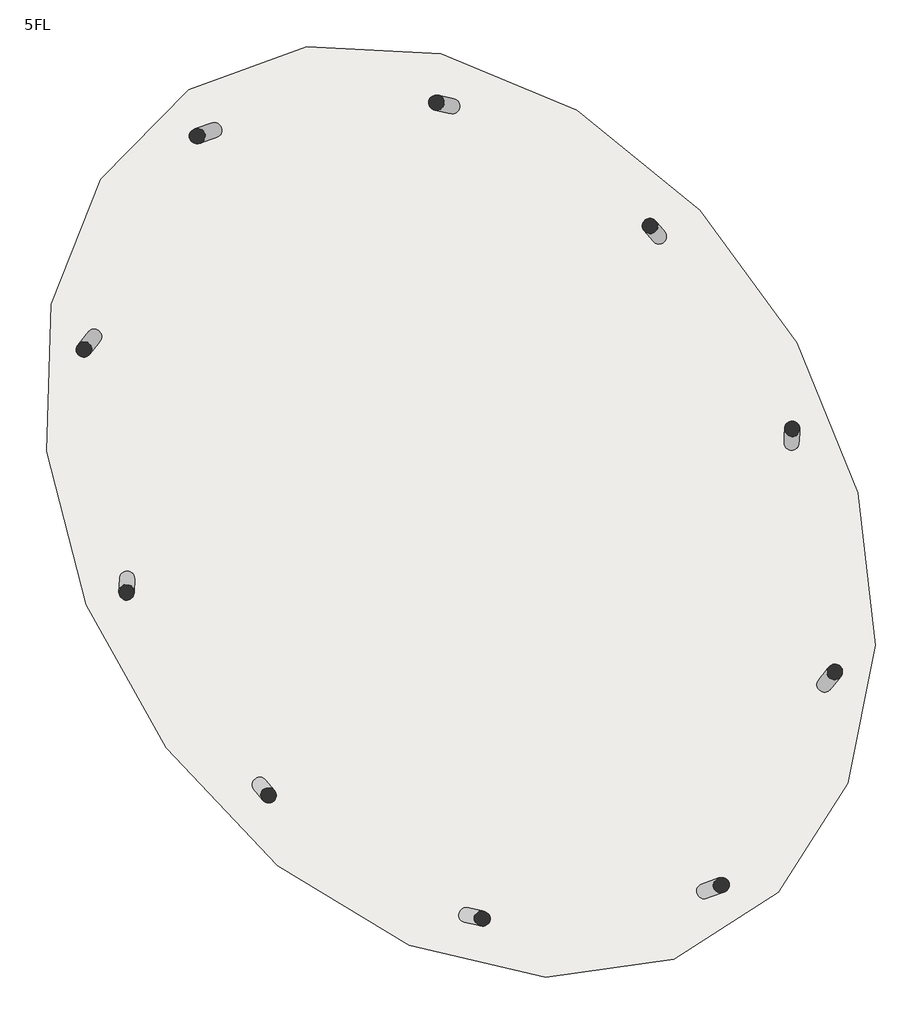
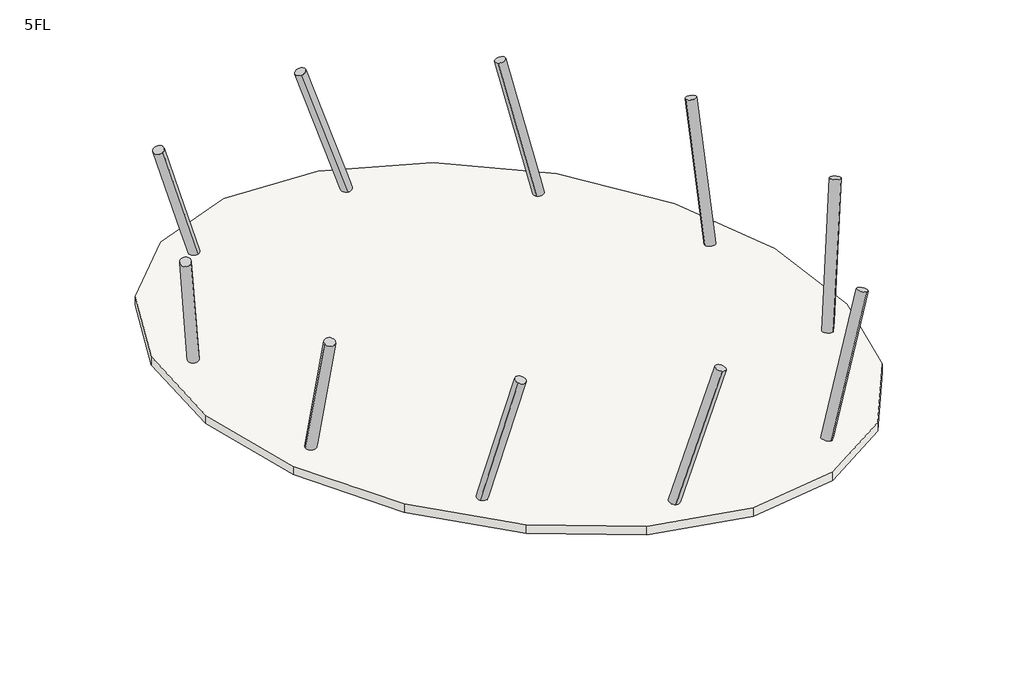
# One storey: 10 columns, 1 slab.
"""IFC4 building model written with IfcOpenShell, lengths in millimetres."""

from ifc_helpers import new_model, si_unit, point, frame, frame_2d, origin, place, context, project, spatial, polyline, circle_curve, trimmed, segment, composite_curve, outline, extrude, element, save

model = new_model("IFC4")

# Units and contexts
model_context = context("Model", 3, world=origin())
ifc_project = project(units=[si_unit("LENGTHUNIT", "METRE", prefix="MILLI")], contexts=[model_context])

# Site, building, storey
site = spatial("IfcSite", under=ifc_project)
building = spatial("IfcBuilding", under=site)
storey = spatial("IfcBuildingStorey", under=building, Name="5FL", Elevation=18000.0)

# Columns
placement = place(None, origin())
element("IfcColumn", 1, ObjectType="コンクリート-円形-柱 : 750", at=placement, inside=storey, context=model_context, shape_type="SweptSolid", body=[
    extrude(outline(composite_curve([segment(trimmed(circle_curve(frame_2d((0.0, -175.0000001)), 175.0), [point((0.0, -350.0000001))], [point((0.0, 0.0))], False, "CARTESIAN"), True, "CONTINUOUS"), segment(trimmed(circle_curve(frame_2d((0.0, -175.0000001)), 175.0), [point((0.0, 0.0))], [point((0.0, -350.0000001))], False, "CARTESIAN"), True, "CONTINUOUS")], self_intersect=False)), frame((-5595.8820356, 8632.5549364, 18000.0), z_axis=(-0.3160724442393226, -0.11108929791393882, 0.9422087761645868), x_axis=(-0.8889040361904681, -0.31242117778067396, -0.3350263006368777)), (0.0, 0.0, 1.0), 4776.0115527),
])
element("IfcColumn", 2, ObjectType="コンクリート-円形-柱 : 750", at=placement, inside=storey, context=model_context, shape_type="SweptSolid", body=[
    extrude(outline(composite_curve([segment(trimmed(circle_curve(frame_2d((0.0, -175.0)), 175.0), [point((0.0, -350.0))], [point((0.0, 0.0))], False, "CARTESIAN"), True, "CONTINUOUS"), segment(trimmed(circle_curve(frame_2d((0.0, -175.0)), 175.0), [point((0.0, 0.0))], [point((0.0, -350.0))], False, "CARTESIAN"), True, "CONTINUOUS")], self_intersect=False)), frame((-8300.1966174, 3915.2551119, 18000.0), z_axis=(-0.19134437507856675, -0.23607455338716757, 0.952709890453984), x_axis=(-0.5998910059272748, -0.7401262840734711, -0.3038813331403524)), (0.0, 0.0, 1.0), 4723.3686194),
])
element("IfcColumn", 3, ObjectType="コンクリート-円形-柱 : 750", at=placement, inside=storey, context=model_context, shape_type="SweptSolid", body=[
    extrude(outline(composite_curve([segment(trimmed(circle_curve(frame_2d((0.0, -174.9999999)), 175.0), [point((1e-07, -350.0))], [point((0.0, 0.0))], False, "CARTESIAN"), True, "CONTINUOUS"), segment(trimmed(circle_curve(frame_2d((0.0, -174.9999999)), 175.0), [point((0.0, 0.0))], [point((1e-07, -350.0))], False, "CARTESIAN"), True, "CONTINUOUS")], self_intersect=False)), frame((-7503.5385113, -1574.7884735, 18000.0), z_axis=(-0.010174401539469679, -0.2585133773793969, 0.9659540958395545), x_axis=(-0.037987983353784824, -0.9652068319225283, -0.25871351864714925)), (0.0, 0.0, 1.0), 4658.6064694),
])
element("IfcColumn", 4, ObjectType="コンクリート-円形-柱 : 750", at=placement, inside=storey, context=model_context, shape_type="SweptSolid", body=[
    extrude(outline(composite_curve([segment(trimmed(circle_curve(frame_2d((1e-07, -175.0)), 175.0), [point((0.0, -350.0))], [point((0.0, 0.0))], False, "CARTESIAN"), True, "CONTINUOUS"), segment(trimmed(circle_curve(frame_2d((1e-07, -175.0)), 175.0), [point((0.0, 0.0))], [point((0.0, -350.0))], False, "CARTESIAN"), True, "CONTINUOUS")], self_intersect=False)), frame((-4481.951061, -6220.6214896, 18000.0), z_axis=(0.16585051662713518, -0.19741327886939466, 0.9661892172139714), x_axis=(0.6214965858800432, -0.7397726658913514, -0.25783404844871255)), (0.0, 0.0, 1.0), 4657.4727984),
])
element("IfcColumn", 5, ObjectType="コンクリート-円形-柱 : 750", at=placement, inside=storey, context=model_context, shape_type="SweptSolid", body=[
    extrude(outline(composite_curve([segment(trimmed(circle_curve(frame_2d((-1e-07, -174.9999999)), 175.0), [point((0.0, -349.9999999))], [point((0.0, 0.0))], False, "CARTESIAN"), True, "CONTINUOUS"), segment(trimmed(circle_curve(frame_2d((-1e-07, -174.9999999)), 175.0), [point((0.0, 0.0))], [point((0.0, -349.9999999))], False, "CARTESIAN"), True, "CONTINUOUS")], self_intersect=False)), frame((195.5067974, -9175.2712794, 18000.0), z_axis=(0.2953258471996599, -0.06630137645773637, 0.9530932648254382), x_axis=(0.9299460730744334, -0.20877517244407529, -0.302676772389933)), (0.0, 0.0, 1.0), 4721.4686802),
])
element("IfcColumn", 6, ObjectType="コンクリート-円形-柱 : 750", at=placement, inside=storey, context=model_context, shape_type="SweptSolid", body=[
    extrude(outline(composite_curve([segment(trimmed(circle_curve(frame_2d((0.0, -175.0000001)), 175.0), [point((0.0, -350.0))], [point((0.0, 0.0))], False, "CARTESIAN"), True, "CONTINUOUS"), segment(trimmed(circle_curve(frame_2d((0.0, -175.0000001)), 175.0), [point((0.0, 0.0))], [point((0.0, -350.0))], False, "CARTESIAN"), True, "CONTINUOUS")], self_intersect=False)), frame((5595.8820724, -8632.5549329, 18000.0), z_axis=(0.3160724441365904, 0.11108929887426984, 0.9422087760858234), x_axis=(0.888904035239524, 0.3124211802487731, -0.3350263008583877)), (0.0, 0.0, 1.0), 4776.0115527),
])
element("IfcColumn", 7, ObjectType="コンクリート-円形-柱 : 750", at=placement, inside=storey, context=model_context, shape_type="SweptSolid", body=[
    extrude(outline(composite_curve([segment(trimmed(circle_curve(frame_2d((0.0, -175.0)), 175.0), [point((0.0, -350.0))], [point((0.0, 0.0))], False, "CARTESIAN"), True, "CONTINUOUS"), segment(trimmed(circle_curve(frame_2d((0.0, -175.0)), 175.0), [point((0.0, 0.0))], [point((0.0, -350.0))], False, "CARTESIAN"), True, "CONTINUOUS")], self_intersect=False)), frame((8300.1966113, -3915.2550865, 18000.0), z_axis=(0.19134437572990706, 0.23607455280450085, 0.9527098904675481), x_axis=(0.5998910080618053, 0.7401262823608402, -0.3038813330978276)), (0.0, 0.0, 1.0), 4723.3686194),
])
element("IfcColumn", 8, ObjectType="コンクリート-円形-柱 : 750", at=placement, inside=storey, context=model_context, shape_type="SweptSolid", body=[
    extrude(outline(composite_curve([segment(trimmed(circle_curve(frame_2d((0.0, -175.0)), 175.0), [point((0.0, -350.0000001))], [point((0.0, 0.0))], False, "CARTESIAN"), True, "CONTINUOUS"), segment(trimmed(circle_curve(frame_2d((0.0, -175.0)), 175.0), [point((0.0, 0.0))], [point((0.0, -350.0000001))], False, "CARTESIAN"), True, "CONTINUOUS")], self_intersect=False)), frame((7503.5384883, 1574.7884899, 18000.0), z_axis=(0.01017440149479294, 0.2585133764783915, 0.9659540960811566), x_axis=(0.03798798332893155, 0.9652068321652956, -0.25871351774508383)), (0.0, 0.0, 1.0), 4658.6064694),
])
element("IfcColumn", 9, ObjectType="コンクリート-円形-柱 : 750", at=placement, inside=storey, context=model_context, shape_type="SweptSolid", body=[
    extrude(outline(composite_curve([segment(trimmed(circle_curve(frame_2d((0.0, -175.0)), 175.0), [point((0.0, -350.0000001))], [point((0.0, 0.0))], False, "CARTESIAN"), True, "CONTINUOUS"), segment(trimmed(circle_curve(frame_2d((0.0, -175.0)), 175.0), [point((0.0, 0.0))], [point((0.0, -350.0000001))], False, "CARTESIAN"), True, "CONTINUOUS")], self_intersect=False)), frame((4481.95109, 6220.6214639, 18000.0), z_axis=(-0.16585051382729254, 0.19741327854709606, 0.9661892177604291), x_axis=(-0.6214965806756345, 0.7397726709773783, -0.2578340464009559)), (0.0, 0.0, 1.0), 4657.4727984),
])
element("IfcColumn", 10, ObjectType="コンクリート-円形-柱 : 750", at=placement, inside=storey, context=model_context, shape_type="SweptSolid", body=[
    extrude(outline(composite_curve([segment(trimmed(circle_curve(frame_2d((1e-07, -175.0)), 175.0), [point((0.0, -350.0))], [point((0.0, 0.0))], False, "CARTESIAN"), True, "CONTINUOUS"), segment(trimmed(circle_curve(frame_2d((1e-07, -175.0)), 175.0), [point((0.0, 0.0))], [point((0.0, -350.0))], False, "CARTESIAN"), True, "CONTINUOUS")], self_intersect=False)), frame((-195.5067212, 9175.2712691, 18000.0), z_axis=(-0.2953258462726247, 0.06630137754078398, 0.953093265037348), x_axis=(-0.9299460724122257, 0.208775176361147, -0.3026767717226539)), (0.0, 0.0, 1.0), 4721.4686802),
])

# Slab
element("IfcSlab", 11, ObjectType="一般 300 mm", at=placement, inside=storey, context=model_context, shape_type="SweptSolid", body=[
    extrude(outline(polyline([(-9428.0004343, 4773.4128834), (-8291.7580013, 7663.867557), (-6249.936122, 9725.0904349), (-3526.7783801, 10726.1340166), (-425.5161627, 10558.9582223), (2715.7498844, 9248.1185765), (5560.2985118, 6939.5038603), (7804.0702115, 3883.1285758), (9206.3920338, 407.6171893), (9615.2780389, -3114.1977627), (8983.0605311, -6303.992306), (7372.3511739, -8815.0936247), (4955.9058348, -10368.0487216), (2002.6148957, -10790.0523336), (-1161.5569269, -10040.0490546), (-4195.2551147, -8205.098477), (-6774.1459202, -5485.7220472), (-8622.2262268, -2175.0513452), (-9540.5478275, 1371.4743126), (-9428.0004343, 4773.4128834)])), frame((0.0, 0.0, 17700.0), z_axis=(0.0, 0.0, 1.0), x_axis=(1.0, 0.0, 0.0)), (0.0, 0.0, 1.0), 300.0),
])

save(model, "model.ifc")

# Revit data of these elements
# Type "コンクリート-円形-柱 : 750"
#   Keynote = "03310.Q1"
#   R = 350 mm
#   Structural Material [instance default] = コンクリート - 現場打ち
# Type "一般 300 mm"
#   Function = 0
#   Layers, outside or top first: 300 mm no material (function 1)
# Elements 1, 2, 3, 4, 5, 6, 7, 8, 9, 10 (IfcColumn, "コンクリート-円形-柱 : 750")
#   Structural Material = コンクリート - 現場打ち
#   Phase Created = 新しい建設
#   Materials on its faces: "コンクリート - 現場打ち"
# Element 11 (IfcSlab, "一般 300 mm")
#   Height Offset From Level = 0 mm
#   Phase Created = 新しい建設
# Materials
#   "コンクリート - 現場打ち": class "コンクリート", colour RGB 192 192 192, transparency 0
